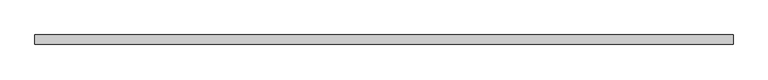
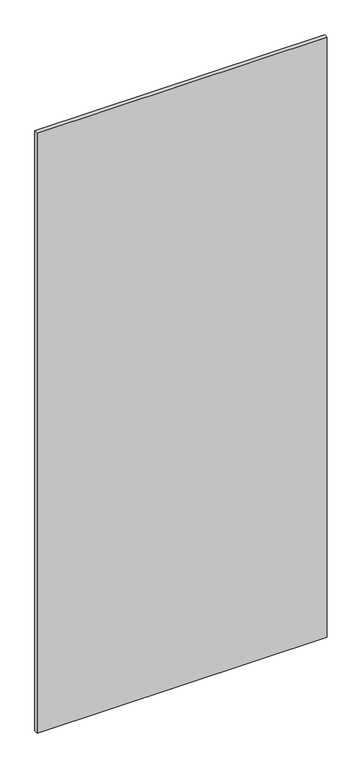
"""IFC4 building model written with IfcOpenShell, lengths in millimetres: plate geometry, 系统嵌板 : 玻璃."""

from ifc_helpers import new_model, si_unit, origin, origin_with_axes, place, context, project, spatial, polyline, outline, extrude, source, transform, mapped, element, save


def plate_0c29ff76(model_context):
    return source(origin(), model_context, "Body", "SweptSolid", [
        extrude(outline(polyline([(915.0, -12.5), (-915.0, -12.5), (-915.0, 12.5), (915.0, 12.5), (915.0, -12.5)])), origin_with_axes(), (0.0, 0.0, 1.0), 4000.0),
    ])


if __name__ == "__main__":
    model = new_model("IFC4")
    model_context = context("Model", 3, world=origin())
    ifc_project = project(units=[si_unit("LENGTHUNIT", "METRE", prefix="MILLI")], contexts=[model_context])
    site = spatial("IfcSite", under=ifc_project)
    building = spatial("IfcBuilding", under=site)
    placement = place(None, origin())
    plate_shape = plate_0c29ff76(model_context)
    element("IfcPlate", 1, ObjectType="系统嵌板 : 玻璃", at=placement, inside=building, context=model_context, shape_type="MappedRepresentation", body=[
        mapped(plate_shape, transform((0.0, 0.0, 0.0), x_axis=(1.0, 0.0, 0.0), y_axis=(0.0, 1.0, 0.0), z_axis=(0.0, 0.0, 1.0))),
    ])
    save(model, "model.ifc")

# Revit data of these elements
# Type "系统嵌板 : 玻璃"
#   Construction Type Id = "GSP4R"
#   Analytic Construction = "1/8 英寸 Pilkington 单层玻璃"
#   Visual Light Transmittance = 0.9
#   Solar Heat Gain Coefficient = 0.86
#   Heat Transfer Coefficient (U) = 6.7069 W/(m²·K)
# Element 1 (IfcPlate, "系统嵌板 : 玻璃")
#   Materials on its faces: "玻璃"
# Materials
#   "玻璃": class "玻璃", colour RGB 0 128 192, transparency 0.9, Description = "钠钙玻璃", Cost = 0
